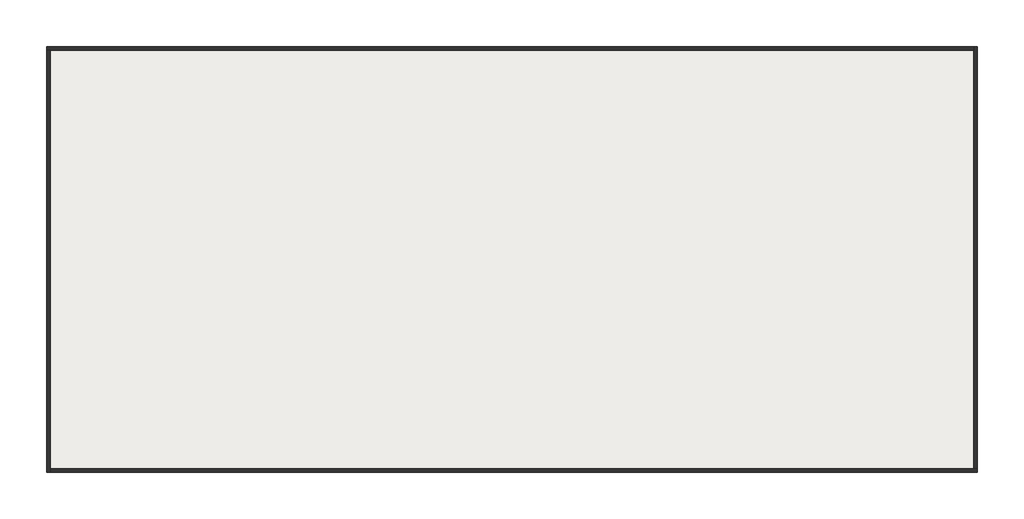
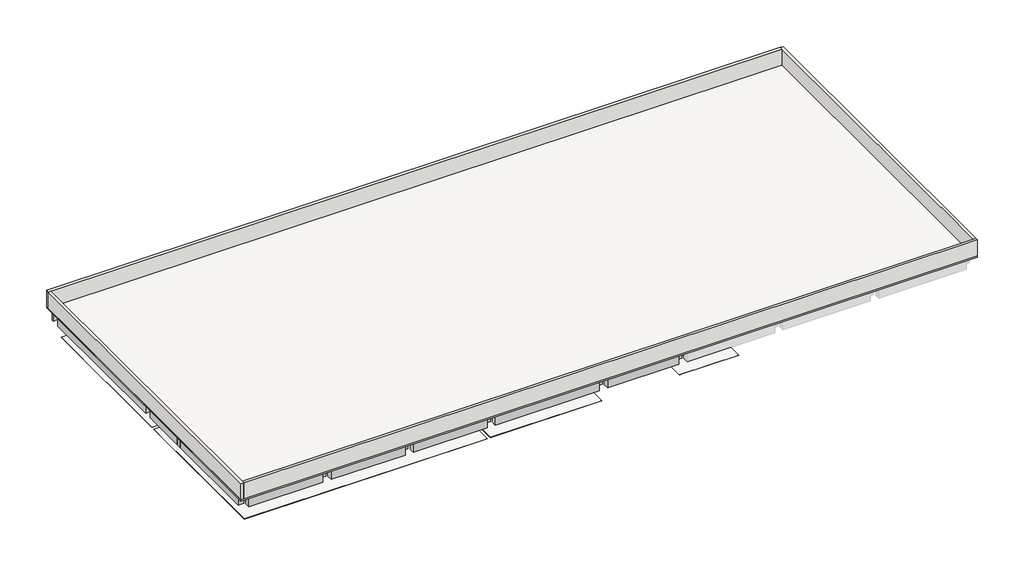
# One storey, part 1 of 2: 25 beams, 16 coverings, 4 walls, 1 roof.
"""IFC4 building model written with IfcOpenShell, lengths in millimetres."""

from ifc_helpers import new_model, si_unit, frame, origin, place, context, project, spatial, polyline, outline, extrude, faceted_brep, element, save

model = new_model("IFC4")

# Units and contexts
model_context = context("Model", 3, world=origin())
ifc_project = project(units=[si_unit("LENGTHUNIT", "METRE", prefix="MILLI")], contexts=[model_context])

# Site, building, storey
site = spatial("IfcSite", under=ifc_project)
building = spatial("IfcBuilding", under=site)
storey = spatial("IfcBuildingStorey", under=building, Name="TOC", Elevation=7650.0)

# Beams
placement = place(None, origin())
element("IfcBeam", 1, ObjectType="RC Beam_Rectangular : H_SB_ACB_B400xH900", at=placement, inside=storey, context=model_context, shape_type="Brep", body=[
    faceted_brep([(224.7, 12116.5208589, 7500.0), (224.7, 12116.5208589, 6750.0), (5624.7, 12116.5208589, 6750.0), (5624.7, 12116.5208589, 7500.0), (5724.7, 12116.5208589, 7500.0), (6124.7, 12116.5208589, 7500.0), (6124.7, 12116.5208589, 7549.0), (5724.7, 12116.5208589, 7549.0), (124.7, 12116.5208589, 7549.0), (-275.3, 12116.5208589, 7549.0), (-275.3, 12116.5208589, 7500.0), (124.7, 12116.5208589, 7500.0), (224.7, 12516.5208589, 6750.0), (5624.7, 12516.5208589, 6750.0), (224.7, 12516.5208589, 7500.0), (124.7, 12516.5208589, 7500.0), (-275.3, 12516.5208589, 7500.0), (-275.3, 12516.5208589, 7549.0), (124.7, 12516.5208589, 7549.0), (5724.7, 12516.5208589, 7549.0), (6124.7, 12516.5208589, 7549.0), (6124.7, 12516.5208589, 7500.0), (5724.7, 12516.5208589, 7500.0), (5624.7, 12516.5208589, 7500.0)], [[[0, 1, 2, 3, 4, 5, 6, 7, 8, 9, 10, 11]], [[1, 12, 13, 2]], [[12, 14, 15, 16, 17, 18, 19, 20, 21, 22, 23, 13]], [[1, 0, 14, 12]], [[0, 11, 10, 16, 15, 14]], [[23, 3, 2, 13]], [[3, 23, 22, 21, 5, 4]], [[9, 8, 7, 6, 20, 19, 18, 17]], [[9, 17, 16, 10]], [[20, 6, 5, 21]]]),
])
element("IfcBeam", 2, ObjectType="RC Beam_Rectangular : H_SB_ACB_B400xH900", at=placement, inside=storey, context=model_context, shape_type="Brep", body=[
    faceted_brep([(6224.7, 12116.5208589, 7500.0), (6224.7, 12116.5208589, 6750.0), (11624.7, 12116.5208589, 6750.0), (11624.7, 12116.5208589, 7500.0), (11724.7, 12116.5208589, 7500.0), (12124.7, 12116.5208589, 7500.0), (12124.7, 12116.5208589, 7549.0), (11724.7, 12116.5208589, 7549.0), (6124.7, 12116.5208589, 7549.0), (6124.7, 12116.5208589, 7500.0), (6224.7, 12516.5208589, 6750.0), (11624.7, 12516.5208589, 6750.0), (6224.7, 12516.5208589, 7500.0), (6124.7, 12516.5208589, 7500.0), (6124.7, 12516.5208589, 7549.0), (11724.7, 12516.5208589, 7549.0), (12124.7, 12516.5208589, 7549.0), (12124.7, 12516.5208589, 7500.0), (11724.7, 12516.5208589, 7500.0), (11624.7, 12516.5208589, 7500.0)], [[[0, 1, 2, 3, 4, 5, 6, 7, 8, 9]], [[1, 10, 11, 2]], [[10, 12, 13, 14, 15, 16, 17, 18, 19, 11]], [[1, 0, 12, 10]], [[0, 9, 13, 12]], [[19, 3, 2, 11]], [[3, 19, 18, 17, 5, 4]], [[8, 7, 6, 16, 15, 14]], [[16, 6, 5, 17]], [[8, 14, 13, 9]]]),
])
element("IfcBeam", 3, ObjectType="RC Beam_Rectangular : H_SB_ACB_B400xH900", at=placement, inside=storey, context=model_context, shape_type="Brep", body=[
    faceted_brep([(12224.7, 12116.5208589, 7500.0), (12224.7, 12116.5208589, 6750.0), (17624.7, 12116.5208589, 6750.0), (17624.7, 12116.5208589, 7500.0), (17724.7, 12116.5208589, 7500.0), (18124.7, 12116.5208589, 7500.0), (18124.7, 12116.5208589, 7549.0), (17724.7, 12116.5208589, 7549.0), (12124.7, 12116.5208589, 7549.0), (12124.7, 12116.5208589, 7500.0), (12224.7, 12516.5208589, 6750.0), (17624.7, 12516.5208589, 6750.0), (12224.7, 12516.5208589, 7500.0), (12124.7, 12516.5208589, 7500.0), (12124.7, 12516.5208589, 7549.0), (17724.7, 12516.5208589, 7549.0), (18124.7, 12516.5208589, 7549.0), (18124.7, 12516.5208589, 7500.0), (17724.7, 12516.5208589, 7500.0), (17624.7, 12516.5208589, 7500.0)], [[[0, 1, 2, 3, 4, 5, 6, 7, 8, 9]], [[1, 10, 11, 2]], [[10, 12, 13, 14, 15, 16, 17, 18, 19, 11]], [[1, 0, 12, 10]], [[0, 9, 13, 12]], [[19, 3, 2, 11]], [[3, 19, 18, 17, 5, 4]], [[8, 7, 6, 16, 15, 14]], [[16, 6, 5, 17]], [[8, 14, 13, 9]]]),
])
element("IfcBeam", 4, ObjectType="RC Beam_Rectangular : H_SB_ACB_B400xH900", at=placement, inside=storey, context=model_context, shape_type="Brep", body=[
    faceted_brep([(26324.7, 12116.5208589, 7549.0), (25924.7, 12116.5208589, 7549.0), (18124.7, 12116.5208589, 7549.0), (18124.7, 12116.5208589, 7500.0), (18224.7, 12116.5208589, 7500.0), (18224.7, 12116.5208589, 6750.0), (25924.7, 12116.5208589, 6750.0), (26324.7, 12116.5208589, 6750.0), (26324.7, 12516.5208589, 6750.0), (18224.7, 12516.5208589, 6750.0), (25924.7, 12516.5208589, 6750.0), (18124.7, 12516.5208589, 7549.0), (25924.7, 12516.5208589, 7549.0), (26324.7, 12516.5208589, 7549.0), (18224.7, 12516.5208589, 7500.0), (18124.7, 12516.5208589, 7500.0)], [[[0, 1, 2, 3, 4, 5, 6, 7]], [[8, 7, 6, 5, 9, 10]], [[11, 12, 13, 8, 10, 9, 14, 15]], [[4, 14, 9, 5]], [[14, 4, 3, 15]], [[2, 1, 0, 13, 12, 11]], [[7, 8, 13, 0]], [[2, 11, 15, 3]]]),
])
element("IfcBeam", 5, ObjectType="RC Beam_Rectangular : H_SB_ACB_B400xH900", at=placement, inside=storey, context=model_context, shape_type="Brep", body=[
    faceted_brep([(-275.3, 8216.5208589, 6750.0), (124.7, 8216.5208589, 6750.0), (5724.7, 8216.5208589, 6750.0), (6124.7, 8216.5208589, 6750.0), (6124.7, 8216.5208589, 7549.0), (5724.7, 8216.5208589, 7549.0), (124.7, 8216.5208589, 7549.0), (-275.3, 8216.5208589, 7549.0), (-275.3, 8616.5208589, 6750.0), (124.7, 8616.5208589, 6750.0), (5724.7, 8616.5208589, 6750.0), (6124.7, 8616.5208589, 6750.0), (-275.3, 8616.5208589, 7549.0), (124.7, 8616.5208589, 7549.0), (5724.7, 8616.5208589, 7549.0), (6124.7, 8616.5208589, 7549.0)], [[[0, 1, 2, 3, 4, 5, 6, 7]], [[0, 8, 9, 10, 11, 3, 2, 1]], [[11, 10, 9, 8, 12, 13, 14, 15]], [[7, 6, 5, 4, 15, 14, 13, 12]], [[8, 0, 7, 12]], [[3, 11, 15, 4]]]),
])
element("IfcBeam", 6, ObjectType="RC Beam_Rectangular : H_SB_ACB_B400xH900", at=placement, inside=storey, context=model_context, shape_type="Brep", body=[
    faceted_brep([(12124.7, 8216.5208589, 6750.0), (12124.7, 8216.5208589, 7549.0), (11724.7, 8216.5208589, 7549.0), (6124.7, 8216.5208589, 7549.0), (6124.7, 8216.5208589, 6750.0), (11724.7, 8216.5208589, 6750.0), (12124.7, 8616.5208589, 6750.0), (6124.7, 8616.5208589, 6750.0), (11724.7, 8616.5208589, 6750.0), (12124.7, 8616.5208589, 7549.0), (6124.7, 8616.5208589, 7549.0), (11724.7, 8616.5208589, 7549.0)], [[[0, 1, 2, 3, 4, 5]], [[6, 0, 5, 4, 7, 8]], [[9, 6, 8, 7, 10, 11]], [[1, 9, 11, 10, 3, 2]], [[0, 6, 9, 1]], [[4, 3, 10, 7]]]),
])
element("IfcBeam", 7, ObjectType="RC Beam_Rectangular : H_SB_ACB_B400xH900", at=placement, inside=storey, context=model_context, shape_type="Brep", body=[
    faceted_brep([(18124.7, 8216.5208589, 6750.0), (18124.7, 8216.5208589, 7549.0), (17724.7, 8216.5208589, 7549.0), (12124.7, 8216.5208589, 7549.0), (12124.7, 8216.5208589, 6750.0), (17724.7, 8216.5208589, 6750.0), (18124.7, 8616.5208589, 6750.0), (12124.7, 8616.5208589, 6750.0), (17724.7, 8616.5208589, 6750.0), (18124.7, 8616.5208589, 7549.0), (12124.7, 8616.5208589, 7549.0), (17724.7, 8616.5208589, 7549.0)], [[[0, 1, 2, 3, 4, 5]], [[6, 0, 5, 4, 7, 8]], [[9, 6, 8, 7, 10, 11]], [[1, 9, 11, 10, 3, 2]], [[0, 6, 9, 1]], [[4, 3, 10, 7]]]),
])
element("IfcBeam", 8, ObjectType="RC Beam_Rectangular : H_SB_ACB_B400xH900", at=placement, inside=storey, context=model_context, shape_type="Brep", body=[
    faceted_brep([(26324.7, 8216.5208589, 7549.0), (25924.7, 8216.5208589, 7549.0), (18124.7, 8216.5208589, 7549.0), (18124.7, 8216.5208589, 6750.0), (25824.7, 8216.5208589, 6750.0), (25824.7, 8216.5208589, 7500.0), (25924.7, 8216.5208589, 7500.0), (26324.7, 8216.5208589, 7500.0), (18124.7, 8616.5208589, 6750.0), (25824.7, 8616.5208589, 6750.0), (18124.7, 8616.5208589, 7549.0), (25924.7, 8616.5208589, 7549.0), (26324.7, 8616.5208589, 7549.0), (26324.7, 8616.5208589, 7500.0), (25924.7, 8616.5208589, 7500.0), (25824.7, 8616.5208589, 7500.0)], [[[0, 1, 2, 3, 4, 5, 6, 7]], [[3, 8, 9, 4]], [[10, 11, 12, 13, 14, 15, 9, 8]], [[15, 5, 4, 9]], [[5, 15, 14, 13, 7, 6]], [[2, 1, 0, 12, 11, 10]], [[12, 0, 7, 13]], [[3, 2, 10, 8]]]),
])
element("IfcBeam", 9, ObjectType="RC Beam_Rectangular : H_SB_ACB_B400xH900", at=placement, inside=storey, context=model_context, shape_type="Brep", body=[
    faceted_brep([(224.7, 416.5208589, 7500.0), (224.7, 416.5208589, 6750.0), (5624.7, 416.5208589, 6750.0), (5624.7, 416.5208589, 7500.0), (6124.7, 416.5208589, 7500.0), (6124.7, 416.5208589, 7549.0), (-275.3, 416.5208589, 7549.0), (-275.3, 416.5208589, 7500.0), (224.7, 816.5208589, 6750.0), (5624.7, 816.5208589, 6750.0), (224.7, 816.5208589, 7500.0), (124.7, 816.5208589, 7500.0), (-275.3, 816.5208589, 7500.0), (-275.3, 816.5208589, 7549.0), (124.7, 816.5208589, 7549.0), (5724.7, 816.5208589, 7549.0), (6124.7, 816.5208589, 7549.0), (6124.7, 816.5208589, 7500.0), (5724.7, 816.5208589, 7500.0), (5624.7, 816.5208589, 7500.0)], [[[0, 1, 2, 3, 4, 5, 6, 7]], [[1, 8, 9, 2]], [[8, 10, 11, 12, 13, 14, 15, 16, 17, 18, 19, 9]], [[8, 1, 0, 10]], [[12, 11, 10, 0, 7]], [[19, 3, 2, 9]], [[3, 19, 18, 17, 4]], [[6, 5, 16, 15, 14, 13]], [[6, 13, 12, 7]], [[16, 5, 4, 17]]]),
])
element("IfcBeam", 10, ObjectType="RC Beam_Rectangular : H_SB_ACB_B400xH900", at=placement, inside=storey, context=model_context, shape_type="Brep", body=[
    faceted_brep([(6224.7, 416.5208589, 7500.0), (6224.7, 416.5208589, 6750.0), (11624.7, 416.5208589, 6750.0), (11624.7, 416.5208589, 7500.0), (12124.7, 416.5208589, 7500.0), (12124.7, 416.5208589, 7549.0), (6124.7, 416.5208589, 7549.0), (6124.7, 416.5208589, 7500.0), (6224.7, 816.5208589, 6750.0), (11624.7, 816.5208589, 6750.0), (6224.7, 816.5208589, 7500.0), (6124.7, 816.5208589, 7500.0), (6124.7, 816.5208589, 7549.0), (11724.7, 816.5208589, 7549.0), (12124.7, 816.5208589, 7549.0), (12124.7, 816.5208589, 7500.0), (11724.7, 816.5208589, 7500.0), (11624.7, 816.5208589, 7500.0)], [[[0, 1, 2, 3, 4, 5, 6, 7]], [[1, 8, 9, 2]], [[8, 10, 11, 12, 13, 14, 15, 16, 17, 9]], [[8, 1, 0, 10]], [[11, 10, 0, 7]], [[17, 3, 2, 9]], [[3, 17, 16, 15, 4]], [[6, 5, 14, 13, 12]], [[14, 5, 4, 15]], [[6, 12, 11, 7]]]),
])
element("IfcBeam", 11, ObjectType="RC Beam_Rectangular : H_SB_ACB_B400xH900", at=placement, inside=storey, context=model_context, shape_type="Brep", body=[
    faceted_brep([(12224.7, 416.5208589, 7500.0), (12224.7, 416.5208589, 6750.0), (17624.7, 416.5208589, 6750.0), (17624.7, 416.5208589, 7500.0), (18124.7, 416.5208589, 7500.0), (18124.7, 416.5208589, 7549.0), (12124.7, 416.5208589, 7549.0), (12124.7, 416.5208589, 7500.0), (12224.7, 816.5208589, 6750.0), (17624.7, 816.5208589, 6750.0), (12224.7, 816.5208589, 7500.0), (12124.7, 816.5208589, 7500.0), (12124.7, 816.5208589, 7549.0), (17724.7, 816.5208589, 7549.0), (18124.7, 816.5208589, 7549.0), (18124.7, 816.5208589, 7500.0), (17724.7, 816.5208589, 7500.0), (17624.7, 816.5208589, 7500.0)], [[[0, 1, 2, 3, 4, 5, 6, 7]], [[1, 8, 9, 2]], [[8, 10, 11, 12, 13, 14, 15, 16, 17, 9]], [[8, 1, 0, 10]], [[11, 10, 0, 7]], [[17, 3, 2, 9]], [[3, 17, 16, 15, 4]], [[6, 5, 14, 13, 12]], [[14, 5, 4, 15]], [[6, 12, 11, 7]]]),
])
element("IfcBeam", 12, ObjectType="RC Beam_Rectangular : H_SB_ACB_B400xH900", at=placement, inside=storey, context=model_context, shape_type="Brep", body=[
    faceted_brep([(18224.7, 416.5208589, 7500.0), (18224.7, 416.5208589, 6750.0), (25824.7, 416.5208589, 6750.0), (25824.7, 416.5208589, 7500.0), (26324.7, 416.5208589, 7500.0), (26324.7, 416.5208589, 7549.0), (18124.7, 416.5208589, 7549.0), (18124.7, 416.5208589, 7500.0), (18224.7, 816.5208589, 6750.0), (25824.7, 816.5208589, 6750.0), (18224.7, 816.5208589, 7500.0), (18124.7, 816.5208589, 7500.0), (18124.7, 816.5208589, 7549.0), (25924.7, 816.5208589, 7549.0), (26324.7, 816.5208589, 7549.0), (26324.7, 816.5208589, 7500.0), (25924.7, 816.5208589, 7500.0), (25824.7, 816.5208589, 7500.0)], [[[0, 1, 2, 3, 4, 5, 6, 7]], [[1, 8, 9, 2]], [[8, 10, 11, 12, 13, 14, 15, 16, 17, 9]], [[8, 1, 0, 10]], [[11, 10, 0, 7]], [[17, 3, 2, 9]], [[3, 17, 16, 15, 4]], [[6, 5, 14, 13, 12]], [[14, 5, 4, 15]], [[6, 12, 11, 7]]]),
])
element("IfcBeam", 13, ObjectType="RC Beam_Rectangular : H_SB_ACB_B400xH900", at=placement, inside=storey, context=model_context, shape_type="Brep", body=[
    faceted_brep([(26424.7, 416.5208589, 7500.0), (26424.7, 416.5208589, 6750.0), (31624.7, 416.5208589, 6750.0), (31624.7, 416.5208589, 7500.0), (32124.7, 416.5208589, 7500.0), (32124.7, 416.5208589, 7549.0), (26324.7, 416.5208589, 7549.0), (26324.7, 416.5208589, 7500.0), (26424.7, 816.5208589, 6750.0), (31624.7, 816.5208589, 6750.0), (26424.7, 816.5208589, 7500.0), (26324.7, 816.5208589, 7500.0), (26324.7, 816.5208589, 7549.0), (31724.7, 816.5208589, 7549.0), (32124.7, 816.5208589, 7549.0), (32124.7, 816.5208589, 7500.0), (31724.7, 816.5208589, 7500.0), (31624.7, 816.5208589, 7500.0)], [[[0, 1, 2, 3, 4, 5, 6, 7]], [[1, 8, 9, 2]], [[8, 10, 11, 12, 13, 14, 15, 16, 17, 9]], [[8, 1, 0, 10]], [[11, 10, 0, 7]], [[17, 3, 2, 9]], [[3, 17, 16, 15, 4]], [[6, 5, 14, 13, 12]], [[14, 5, 4, 15]], [[6, 12, 11, 7]]]),
])
element("IfcBeam", 14, ObjectType="RC Beam_Rectangular : H_SB_ACB_B400xH900", at=placement, inside=storey, context=model_context, shape_type="SweptSolid", body=[
    extrude(outline(polyline([(8216.5208589, 7549.0), (8216.5208589, 6750.0), (916.5208589, 6750.0), (916.5208589, 7500.0), (816.5208589, 7500.0), (816.5208589, 7549.0), (8216.5208589, 7549.0)])), frame((-275.3, 0.0, 0.0), z_axis=(1.0, 0.0, 0.0), x_axis=(0.0, 1.0, 0.0)), (0.0, 0.0, 1.0), 400.0),
])
element("IfcBeam", 15, ObjectType="RC Beam_Rectangular : H_SB_ACB_B400xH900", at=placement, inside=storey, context=model_context, shape_type="SweptSolid", body=[
    extrude(outline(polyline([(8616.5208589, 7549.0), (12116.5208589, 7549.0), (12116.5208589, 7500.0), (12016.5208589, 7500.0), (12016.5208589, 6750.0), (8616.5208589, 6750.0), (8616.5208589, 7549.0)])), frame((-275.3, 0.0, 0.0), z_axis=(1.0, 0.0, 0.0), x_axis=(0.0, 1.0, 0.0)), (0.0, 0.0, 1.0), 400.0),
])
element("IfcBeam", 16, ObjectType="RC Beam_Rectangular : H_SB_ACB_B400xH900", at=placement, inside=storey, context=model_context, shape_type="Brep", body=[
    faceted_brep([(124.7, 24429.2208589, 6750.0), (-275.3, 24429.2208589, 6750.0), (-275.3, 24429.2208589, 7549.0), (124.7, 24429.2208589, 7549.0), (124.7, 12616.5208589, 7500.0), (124.7, 12616.5208589, 6750.0), (124.7, 23716.5208589, 6750.0), (124.7, 23716.5208589, 7500.0), (124.7, 23816.5208589, 7500.0), (124.7, 24216.5208589, 7500.0), (124.7, 24316.5208589, 7500.0), (124.7, 24316.5208589, 6750.0), (124.7, 24216.5208589, 7549.0), (124.7, 23816.5208589, 7549.0), (124.7, 12516.5208589, 7549.0), (124.7, 12516.5208589, 7500.0), (-275.3, 24316.5208589, 6750.0), (-275.3, 12616.5208589, 6750.0), (-275.3, 12616.5208589, 7500.0), (-275.3, 12516.5208589, 7500.0), (-275.3, 12516.5208589, 7549.0), (-275.3, 24316.5208589, 7500.0), (-275.3, 23716.5208589, 7500.0), (-275.3, 23716.5208589, 6750.0)], [[[0, 1, 2, 3]], [[4, 5, 6, 7, 8, 9, 10, 11, 0, 3, 12, 13, 14, 15]], [[1, 0, 11, 16]], [[17, 18, 19, 20, 2, 1, 16, 21, 22, 23]], [[19, 15, 14, 20]], [[5, 4, 18, 17]], [[4, 15, 19, 18]], [[22, 7, 6, 23]], [[7, 22, 21, 10, 9, 8]], [[3, 2, 20, 14, 13, 12]], [[10, 21, 16, 11]], [[5, 17, 23, 6]]]),
])
element("IfcBeam", 17, ObjectType="RC Beam_Rectangular : H_SB_ACB_B400xH900", at=placement, inside=storey, context=model_context, shape_type="SweptSolid", body=[
    extrude(outline(polyline([(8216.5208589, 7549.0), (8216.5208589, 6750.0), (916.5208589, 6750.0), (916.5208589, 7500.0), (816.5208589, 7500.0), (816.5208589, 7549.0), (8216.5208589, 7549.0)])), frame((5724.7, 0.0, 0.0), z_axis=(1.0, 0.0, 0.0), x_axis=(0.0, 1.0, 0.0)), (0.0, 0.0, 1.0), 400.0),
])
element("IfcBeam", 18, ObjectType="RC Beam_Rectangular : H_SB_ACB_B400xH900", at=placement, inside=storey, context=model_context, shape_type="SweptSolid", body=[
    extrude(outline(polyline([(8616.5208589, 6750.0), (8616.5208589, 7549.0), (12116.5208589, 7549.0), (12116.5208589, 7500.0), (12016.5208589, 7500.0), (12016.5208589, 6750.0), (8616.5208589, 6750.0)])), frame((5724.7, 0.0, 0.0), z_axis=(1.0, 0.0, 0.0), x_axis=(0.0, 1.0, 0.0)), (0.0, 0.0, 1.0), 400.0),
])
element("IfcBeam", 19, ObjectType="RC Beam_Rectangular : H_SB_ACB_B400xH900", at=placement, inside=storey, context=model_context, shape_type="SweptSolid", body=[
    extrude(outline(polyline([(8216.5208589, 7549.0), (8216.5208589, 6750.0), (916.5208589, 6750.0), (916.5208589, 7500.0), (816.5208589, 7500.0), (816.5208589, 7549.0), (8216.5208589, 7549.0)])), frame((11724.7, 0.0, 0.0), z_axis=(1.0, 0.0, 0.0), x_axis=(0.0, 1.0, 0.0)), (0.0, 0.0, 1.0), 400.0),
])
element("IfcBeam", 20, ObjectType="RC Beam_Rectangular : H_SB_ACB_B400xH900", at=placement, inside=storey, context=model_context, shape_type="SweptSolid", body=[
    extrude(outline(polyline([(8616.5208589, 6750.0), (8616.5208589, 7549.0), (12116.5208589, 7549.0), (12116.5208589, 7500.0), (12016.5208589, 7500.0), (12016.5208589, 6750.0), (8616.5208589, 6750.0)])), frame((11724.7, 0.0, 0.0), z_axis=(1.0, 0.0, 0.0), x_axis=(0.0, 1.0, 0.0)), (0.0, 0.0, 1.0), 400.0),
])
element("IfcBeam", 21, ObjectType="RC Beam_Rectangular : H_SB_ACB_B400xH900", at=placement, inside=storey, context=model_context, shape_type="SweptSolid", body=[
    extrude(outline(polyline([(8216.5208589, 7549.0), (8216.5208589, 6750.0), (916.5208589, 6750.0), (916.5208589, 7500.0), (816.5208589, 7500.0), (816.5208589, 7549.0), (8216.5208589, 7549.0)])), frame((17724.7, 0.0, 0.0), z_axis=(1.0, 0.0, 0.0), x_axis=(0.0, 1.0, 0.0)), (0.0, 0.0, 1.0), 400.0),
])
element("IfcBeam", 22, ObjectType="RC Beam_Rectangular : H_SB_ACB_B400xH900", at=placement, inside=storey, context=model_context, shape_type="SweptSolid", body=[
    extrude(outline(polyline([(8616.5208589, 6750.0), (8616.5208589, 7549.0), (12116.5208589, 7549.0), (12116.5208589, 7500.0), (12016.5208589, 7500.0), (12016.5208589, 6750.0), (8616.5208589, 6750.0)])), frame((17724.7, 0.0, 0.0), z_axis=(1.0, 0.0, 0.0), x_axis=(0.0, 1.0, 0.0)), (0.0, 0.0, 1.0), 400.0),
])
element("IfcBeam", 23, ObjectType="RC Beam_Rectangular : H_SB_ACB_B400xH900", at=placement, inside=storey, context=model_context, shape_type="SweptSolid", body=[
    extrude(outline(polyline([(8116.5208589, 7500.0), (8116.5208589, 6750.0), (916.5208589, 6750.0), (916.5208589, 7500.0), (816.5208589, 7500.0), (816.5208589, 7549.0), (8216.5208589, 7549.0), (8216.5208589, 7500.0), (8116.5208589, 7500.0)])), frame((25924.7, 0.0, 0.0), z_axis=(1.0, 0.0, 0.0), x_axis=(0.0, 1.0, 0.0)), (0.0, 0.0, 1.0), 400.0),
])
element("IfcBeam", 24, ObjectType="RC Beam_Rectangular : H_SB_ACB_B400xH900", at=placement, inside=storey, context=model_context, shape_type="SweptSolid", body=[
    extrude(outline(polyline([(12116.5208589, 7549.0), (12116.5208589, 6750.0), (8716.5208589, 6750.0), (8716.5208589, 7500.0), (8616.5208589, 7500.0), (8616.5208589, 7549.0), (12116.5208589, 7549.0)])), frame((25924.7, 0.0, 0.0), z_axis=(1.0, 0.0, 0.0), x_axis=(0.0, 1.0, 0.0)), (0.0, 0.0, 1.0), 400.0),
])
element("IfcBeam", 25, ObjectType="RC Beam_Rectangular : H_SB_ACB_B400xH900", at=placement, inside=storey, context=model_context, shape_type="SweptSolid", body=[
    extrude(outline(polyline([(8116.5208589, 7500.0), (8116.5208589, 6750.0), (916.5208589, 6750.0), (916.5208589, 7500.0), (816.5208589, 7500.0), (816.5208589, 7549.0), (8216.5208589, 7549.0), (8216.5208589, 7500.0), (8116.5208589, 7500.0)])), frame((31724.7, 0.0, 0.0), z_axis=(1.0, 0.0, 0.0), x_axis=(0.0, 1.0, 0.0)), (0.0, 0.0, 1.0), 400.0),
])

# Coverings
element("IfcCovering", 26, ObjectType="CE741_Acoustic Tiled Ceiling System_600x600x9t_T_bar", at=placement, inside=storey, context=model_context, shape_type="SweptSolid", body=[
    extrude(outline(polyline([(54.7, 23886.5208589), (17807.7, 23886.5208589), (17807.7, 12433.5208589), (54.7, 12433.5208589), (54.7, 23886.5208589)])), frame((0.0, 0.0, 5650.0), z_axis=(0.0, 0.0, 1.0), x_axis=(1.0, 0.0, 0.0)), (0.0, 0.0, 1.0), 9.0),
])
element("IfcCovering", 27, ObjectType="CE741_Acoustic Tiled Ceiling System_600x600x9t_T_bar", at=placement, inside=storey, context=model_context, shape_type="SweptSolid", body=[
    extrude(outline(polyline([(18041.7, 8533.5208589), (18041.7, 23886.5208589), (33157.7, 23886.5208589), (33157.7, 8533.5208589), (18041.7, 8533.5208589)])), frame((0.0, 0.0, 5650.0), z_axis=(0.0, 0.0, 1.0), x_axis=(1.0, 0.0, 0.0)), (0.0, 0.0, 1.0), 9.0),
])
element("IfcCovering", 28, ObjectType="CE741_Acoustic Tiled Ceiling System_600x600x9t_T_bar", at=placement, inside=storey, context=model_context, shape_type="SweptSolid", body=[
    extrude(outline(polyline([(54.7, 746.5208589), (54.7, 12199.5208589), (17807.7, 12199.5208589), (17807.7, 746.5208589), (54.7, 746.5208589)])), frame((0.0, 0.0, 5650.0), z_axis=(0.0, 0.0, 1.0), x_axis=(1.0, 0.0, 0.0)), (0.0, 0.0, 1.0), 9.0),
])
element("IfcCovering", 29, ObjectType="CE741_Acoustic Tiled Ceiling System_600x600x9t_T_bar", at=placement, inside=storey, context=model_context, shape_type="SweptSolid", body=[
    extrude(outline(polyline([(26190.7, 746.5208589), (18041.7, 746.5208589), (18041.7, 8299.5208589), (26190.7, 8299.5208589), (26190.7, 746.5208589)])), frame((0.0, 0.0, 5650.0), z_axis=(0.0, 0.0, 1.0), x_axis=(1.0, 0.0, 0.0)), (0.0, 0.0, 1.0), 9.0),
])
element("IfcCovering", 30, ObjectType="CE741_Acoustic Tiled Ceiling System_600x600x9t_T_bar", at=placement, inside=storey, context=model_context, shape_type="SweptSolid", body=[
    extrude(outline(polyline([(33391.7, 8533.5208589), (33391.7, 23886.5208589), (43607.7, 23886.5208589), (43607.7, 11083.5208589), (36207.7, 11083.5208589), (36207.7, 8533.5208589), (33391.7, 8533.5208589)])), frame((0.0, 0.0, 5650.0), z_axis=(0.0, 0.0, 1.0), x_axis=(1.0, 0.0, 0.0)), (0.0, 0.0, 1.0), 9.0),
])
element("IfcCovering", 31, ObjectType="CE741_Acoustic Tiled Ceiling System_600x600x9t_T_bar", at=placement, inside=storey, context=model_context, shape_type="SweptSolid", body=[
    extrude(outline(polyline([(54.7, 746.5208589), (54.7, 12199.5208589), (17807.7, 12199.5208589), (17807.7, 746.5208589), (54.7, 746.5208589)])), frame((0.0, 0.0, 5650.0), z_axis=(0.0, 0.0, 1.0), x_axis=(1.0, 0.0, 0.0)), (0.0, 0.0, 1.0), 9.0),
])
element("IfcCovering", 32, ObjectType="CE741_Acoustic Tiled Ceiling System_600x600x9t_T_bar", at=placement, inside=storey, context=model_context, shape_type="SweptSolid", body=[
    extrude(outline(polyline([(54.7, 23886.5208589), (17807.7, 23886.5208589), (17807.7, 12433.5208589), (54.7, 12433.5208589), (54.7, 23886.5208589)])), frame((0.0, 0.0, 5650.0), z_axis=(0.0, 0.0, 1.0), x_axis=(1.0, 0.0, 0.0)), (0.0, 0.0, 1.0), 9.0),
])
element("IfcCovering", 33, ObjectType="CE741_Acoustic Tiled Ceiling System_600x600x9t_T_bar", at=placement, inside=storey, context=model_context, shape_type="SweptSolid", body=[
    extrude(outline(polyline([(18041.7, 8533.5208589), (18041.7, 23886.5208589), (33157.7, 23886.5208589), (33157.7, 8533.5208589), (18041.7, 8533.5208589)])), frame((0.0, 0.0, 5650.0), z_axis=(0.0, 0.0, 1.0), x_axis=(1.0, 0.0, 0.0)), (0.0, 0.0, 1.0), 9.0),
])
element("IfcCovering", 34, ObjectType="CE741_Acoustic Tiled Ceiling System_600x600x9t_T_bar", at=placement, inside=storey, context=model_context, shape_type="SweptSolid", body=[
    extrude(outline(polyline([(26190.7, 746.5208589), (18041.7, 746.5208589), (18041.7, 8299.5208589), (26190.7, 8299.5208589), (26190.7, 746.5208589)])), frame((0.0, 0.0, 5650.0), z_axis=(0.0, 0.0, 1.0), x_axis=(1.0, 0.0, 0.0)), (0.0, 0.0, 1.0), 9.0),
])
element("IfcCovering", 35, ObjectType="CE741_Acoustic Tiled Ceiling System_600x600x9t_T_bar", at=placement, inside=storey, context=model_context, shape_type="SweptSolid", body=[
    extrude(outline(polyline([(26424.7, 2880.5208589), (26424.7, 8299.5208589), (28824.7, 8299.5208589), (28824.7, 2880.5208589), (26424.7, 2880.5208589)])), frame((0.0, 0.0, 5650.0), z_axis=(0.0, 0.0, 1.0), x_axis=(1.0, 0.0, 0.0)), (0.0, 0.0, 1.0), 9.0),
])
element("IfcCovering", 36, ObjectType="CE741_Acoustic Tiled Ceiling System_600x600x9t_T_bar", at=placement, inside=storey, context=model_context, shape_type="SweptSolid", body=[
    extrude(outline(polyline([(33391.7, 8533.5208589), (33391.7, 23886.5208589), (43607.7, 23886.5208589), (43607.7, 11083.5208589), (36207.7, 11083.5208589), (36207.7, 8533.5208589), (33391.7, 8533.5208589)])), frame((0.0, 0.0, 5650.0), z_axis=(0.0, 0.0, 1.0), x_axis=(1.0, 0.0, 0.0)), (0.0, 0.0, 1.0), 9.0),
])
element("IfcCovering", 37, ObjectType="CE741_Acoustic Tiled Ceiling System_600x600x9t_T_bar", at=placement, inside=storey, context=model_context, shape_type="SweptSolid", body=[
    extrude(outline(polyline([(38807.7, 3380.5208589), (36441.7, 3380.5208589), (36441.7, 10849.5208589), (45807.7, 10849.5208589), (45807.7, 9899.5208589), (49977.7, 9899.5208589), (49977.7, 10499.5208589), (50660.7, 10499.5208589), (50660.7, 8533.5208589), (45124.7, 8533.5208589), (45124.7, 8299.5208589), (45175.8778017, 8299.5208589), (45175.8778017, 6933.5208589), (43341.7, 6933.5208589), (43341.7, 8533.5208589), (38807.7, 8533.5208589), (38807.7, 3380.5208589)])), frame((0.0, 0.0, 5650.0), z_axis=(0.0, 0.0, 1.0), x_axis=(1.0, 0.0, 0.0)), (0.0, 0.0, 1.0), 9.0),
])
element("IfcCovering", 38, ObjectType="CE741_Acoustic Tiled Ceiling System_600x600x9t_T_bar", at=placement, inside=storey, context=model_context, shape_type="SweptSolid", body=[
    extrude(outline(polyline([(36207.7, 746.5208589), (31858.7, 746.5208589), (31858.7, 8299.5208589), (36207.7, 8299.5208589), (36207.7, 746.5208589)])), frame((0.0, 0.0, 5650.0), z_axis=(0.0, 0.0, 1.0), x_axis=(1.0, 0.0, 0.0)), (0.0, 0.0, 1.0), 9.0),
])
element("IfcCovering", 39, ObjectType="CE741_Acoustic Tiled Ceiling System_600x600x9t_T_bar", at=placement, inside=storey, context=model_context, shape_type="SweptSolid", body=[
    extrude(outline(polyline([(52794.7, 14049.5208589), (52794.7, 11967.5208589), (50660.7, 11967.5208589), (50660.7, 10733.5208589), (49743.7, 10733.5208589), (49743.7, 10133.5208589), (46041.7, 10133.5208589), (46041.7, 14049.5208589), (52794.7, 14049.5208589)])), frame((0.0, 0.0, 5650.0), z_axis=(0.0, 0.0, 1.0), x_axis=(1.0, 0.0, 0.0)), (0.0, 0.0, 1.0), 9.0),
])
element("IfcCovering", 40, ObjectType="CE741_Acoustic Tiled Ceiling System_600x600x9t_T_bar", at=placement, inside=storey, context=model_context, shape_type="SweptSolid", body=[
    extrude(outline(polyline([(52794.7, 18549.5208589), (52794.7, 14283.5208589), (48441.7, 14283.5208589), (48441.7, 17180.5208589), (46041.7, 17180.5208589), (46041.7, 18549.5208589), (52794.7, 18549.5208589)])), frame((0.0, 0.0, 5650.0), z_axis=(0.0, 0.0, 1.0), x_axis=(1.0, 0.0, 0.0)), (0.0, 0.0, 1.0), 9.0),
])
element("IfcCovering", 41, ObjectType="CE741_Acoustic Tiled Ceiling System_600x600x9t_T_bar", at=placement, inside=storey, context=model_context, shape_type="SweptSolid", body=[
    extrude(outline(polyline([(49041.7, 19949.5208589), (49041.7, 23886.5208589), (52794.7, 23886.5208589), (52794.7, 18783.5208589), (47658.7, 18783.5208589), (47658.7, 19949.5208589), (49041.7, 19949.5208589)])), frame((0.0, 0.0, 5650.0), z_axis=(0.0, 0.0, 1.0), x_axis=(1.0, 0.0, 0.0)), (0.0, 0.0, 1.0), 9.0),
])

# Roof
element("IfcRoof", 42, ObjectType="H_RF_AMF_RC Roof Finish_WP_Insulation_Protection", at=placement, inside=storey, context=model_context, shape_type="SweptSolid", body=[
    extrude(outline(polyline([(53324.7, 24816.5208589), (53324.7, 216.5208589), (-475.3, 216.5208589), (-475.3, 24816.5208589), (53324.7, 24816.5208589)])), frame((0.0, 0.0, 7549.0), z_axis=(0.0, 0.0, 1.0), x_axis=(1.0, 0.0, 0.0)), (0.0, 0.0, 1.0), 101.0),
])

# Walls
element("IfcWall", 43, ObjectType="H_WA_AMW_RC Wall_T200 (No Finish)", at=placement, inside=storey, context=model_context, shape_type="Brep", body=[
    faceted_brep([(-475.3, 24616.5208589, 7650.0), (-275.3, 24616.5208589, 7650.0), (53124.7, 24616.5208589, 7650.0), (53124.7, 24616.5208589, 8900.0), (-275.3, 24616.5208589, 8900.0), (-475.3, 24616.5208589, 8900.0), (-475.3, 24816.5208589, 7650.0), (-475.3, 24816.5208589, 8900.0), (53124.7, 24816.5208589, 8900.0), (53124.7, 24816.5208589, 7650.0)], [[[0, 1, 2, 3, 4, 5]], [[6, 7, 8, 9]], [[2, 1, 0, 6, 9]], [[5, 4, 3, 8, 7]], [[0, 5, 7, 6]], [[3, 2, 9, 8]]]),
])
element("IfcWall", 44, ObjectType="H_WA_AMW_RC Wall_T200 (No Finish)", at=placement, inside=storey, context=model_context, shape_type="Brep", body=[
    faceted_brep([(-275.3, 216.5208589, 7650.0), (-275.3, 416.5208589, 7650.0), (-275.3, 24616.5208589, 7650.0), (-275.3, 24616.5208589, 8900.0), (-275.3, 416.5208589, 8900.0), (-275.3, 216.5208589, 8900.0), (-475.3, 216.5208589, 7650.0), (-475.3, 216.5208589, 8900.0), (-475.3, 24616.5208589, 8900.0), (-475.3, 24616.5208589, 7650.0)], [[[0, 1, 2, 3, 4, 5]], [[6, 7, 8, 9]], [[2, 1, 0, 6, 9]], [[5, 4, 3, 8, 7]], [[0, 5, 7, 6]], [[3, 2, 9, 8]]]),
])
element("IfcWall", 45, ObjectType="H_WA_AMW_RC Wall_T200 (No Finish)", at=placement, inside=storey, context=model_context, shape_type="Brep", body=[
    faceted_brep([(53324.7, 416.5208589, 7650.0), (53124.7, 416.5208589, 7650.0), (-275.3, 416.5208589, 7650.0), (-275.3, 416.5208589, 8900.0), (53124.7, 416.5208589, 8900.0), (53324.7, 416.5208589, 8900.0), (53324.7, 216.5208589, 7650.0), (53324.7, 216.5208589, 8900.0), (-275.3, 216.5208589, 8900.0), (-275.3, 216.5208589, 7650.0)], [[[0, 1, 2, 3, 4, 5]], [[6, 7, 8, 9]], [[2, 1, 0, 6, 9]], [[5, 4, 3, 8, 7]], [[0, 5, 7, 6]], [[3, 2, 9, 8]]]),
])
element("IfcWall", 46, ObjectType="H_WA_AMW_RC Wall_T200 (No Finish)", at=placement, inside=storey, context=model_context, shape_type="Brep", body=[
    faceted_brep([(53124.7, 24816.5208589, 7650.0), (53124.7, 24616.5208589, 7650.0), (53124.7, 416.5208589, 7650.0), (53124.7, 416.5208589, 8900.0), (53124.7, 24616.5208589, 8900.0), (53124.7, 24816.5208589, 8900.0), (53324.7, 24816.5208589, 7650.0), (53324.7, 24816.5208589, 8900.0), (53324.7, 416.5208589, 8900.0), (53324.7, 416.5208589, 7650.0)], [[[0, 1, 2, 3, 4, 5]], [[6, 7, 8, 9]], [[2, 1, 0, 6, 9]], [[5, 4, 3, 8, 7]], [[0, 5, 7, 6]], [[3, 2, 9, 8]]]),
])

save(model, "model.ifc")

# Revit data of these elements
# Project information
#   Building Name = "SULFUR LOADING CONTROL BD"
#   Project Status = "Project Status"
#   Client Name = "현대엔지니어링"
#   Project Address = "서울시 종로구 율곡로 75(계동)"
#   Project Number = "-"
# Grids (mm)
#   "Y1": line (-3935.398, 24016.521) -> (58968.688, 24016.521)
#   "X1": line (-75.3, 29394.337) -> (-75.3, -4379.638)
#   "X2": line (5924.7, 29394.337) -> (5924.7, -4379.638)
#   "Y3": line (-3935.398, 8416.521) -> (58968.688, 8416.521)
#   "Y4": line (-3935.398, 616.521) -> (58968.688, 616.521)
#   "X3": line (11924.7, 29394.337) -> (11924.7, -4379.638)
#   "X4": line (17924.7, 29394.337) -> (17924.7, -4379.638)
#   "X5": line (26124.7, 29394.337) -> (26124.7, -4379.638)
#   "X6": line (31924.7, 29394.337) -> (31924.7, -4379.638)
#   "X7": line (38924.7, 29394.337) -> (38924.7, -4379.638)
#   "X8": line (45924.7, 29394.337) -> (45924.7, -4379.638)
#   "X9": line (52924.7, 29394.337) -> (52924.7, -4379.638)
#   "X15": line (43724.7, 27041.858) -> (43724.7, 9156.488)
#   "X16": line (36324.7, 27041.858) -> (36324.7, 9156.488)
#   "X17": line (34685.051, 10966.521) -> (55094.626, 10966.521)
#   "X18": line (34685.051, 18666.521) -> (55094.626, 18666.521)
#   "Y2": line (-3935.398, 12316.521) -> (58968.688, 12316.521)
# Type "RC Beam_Rectangular : H_SB_ACB_B400xH900"
#   중앙부 하부근 = ""
#   중앙부 상부근 = ""
#   중앙부 보조근 = ""
#   중앙부 늑근 = ""
#   외단부 하부근 = ""
#   외단부 상부근 = ""
#   외단부 보조근 = ""
#   외단부 늑근 = ""
#   부호 = "TG3"
#   내단부 하부근 = ""
#   내단부 상부근 = ""
#   내단부 보조근 = ""
#   내단부 늑근 = ""
#   ALL 하부근 = "3-D20"
#   ALL 상부근 = "3-D20"
#   ALL 보조근 = ""
#   ALL 늑근 = "2-D10 @120"
#   Width = 400.000 mm
#   Height = 900.000 mm
#   Length [instance default] = 1524.000 mm
#   b = 400.000 mm
#   h = 900.000 mm
#   hec_material3 [instance default] = none
#   hec_material2 [instance default] = none
#   hec_material1 [instance default] = none
#   Structural Material [instance default] = none
#   Assembly Code = ""
# Type "CE741_Acoustic Tiled Ceiling System_600x600x9t_T_bar"
#   built-in parameter 1002203 = 1 (stored number, unit not read)
#   built-in parameter 1002202 = 1 (stored number, unit not read)
#   Layers, outside or top first: 9.000 mm no material (function 4)
# Type "H_RF_AMF_RC Roof Finish_WP_Insulation_Protection"
#   Layers, outside or top first: 50.000 mm no material (function 4); 0.000 mm no material (function 100); 50.000 mm no material (function 3); 1.000 mm no material (function 2)
# Type "H_WA_AMW_RC Wall_T200 (No Finish)"
#   Type Comments = ""
#   Layers, outside or top first: 0.000 mm no material (function 100); 0.000 mm no material (function 100); 200.000 mm no material (function 1); 0.000 mm no material (function 100); 0.000 mm no material (function 100); 0.000 mm no material (function 100)
# Elements 1, 2, 3, 4, 5, 6, 7, 8, 9, 10, 11, 12, 13, 14, 15, 16, 17, 18, 19, 20, 21, 22, 23, 24, 25 (IfcBeam, "RC Beam_Rectangular : H_SB_ACB_B400xH900")
#   hec_material3 = none
#   hec_material2 = none
#   hec_material1 = none
#   Structural Material = none
#   Phase Created = New Construction
# Elements 26, 27, 28, 29, 30, 31, 32, 33, 34, 35, 36, 37, 38, 39, 40, 41 (IfcCovering, "CE741_Acoustic Tiled Ceiling System_600x600x9t_T_bar")
#   Height Offset From Level = -2000.000 mm
#   Phase Created = New Construction
# Element 42 (IfcRoof, "H_RF_AMF_RC Roof Finish_WP_Insulation_Protection")
#   Mark = "RF1"
#   Roof Style Name = "Lightweight Concrete(Slope)+Insulation+Waterproofing+Gravel"
#   Roof Ref. = ""
#   Roof Base Material = "Concrete Slab"
#   Roof Finish_1 = "Light-Weight Concrete Screed (Slope 1%)"
#   Roof Finish_2 = ""
#   Roof Finish_3 = "Rigid Extruded Polystyrene Foam Insulation(XPS)"
#   Roof Finish_4 = "Waterproofing Membrane-EPDM(or Equivalent)"
#   Roof Finish_5 = "Gravel for Roof"
#   built-in parameter 1001705 = 25.0984 (stored number, unit not read)
#   built-in parameter 1001701 = -0.331365 (stored number, unit not read)
#   built-in parameter 1001710 = 33615
#   Roof Style = RF13
#   Phase Created = New Construction
#   Materials on its faces: "Default Roof"
# Element 43 (IfcWall, "H_WA_AMW_RC Wall_T200 (No Finish)")
#   Mark = "PW1"
#   Wall Loca = "ROOF"
#   Wall Style Name = "Concrete Wall+Acrylic Emulsion Paint on Cement Plaster"
#   Wall Ref. = ""
#   Wall Base Material-1 = ""
#   Wall Base Material-2 = ""
#   Wall Base Material-3 = "Concrete Wall"
#   Wall Finish-Ex = "Acrylic Emulsion Paint on Fair Faced Concrete"
#   Top Offset = 0.000 mm
#   Base Offset = 0.000 mm
#   wall height = 1250.000 mm
#   Wall Style No = EW51
#   Phase Created = New Construction
#   Base Constraint = TOC
#   Top Constraint = TOP
#   Materials on its faces: "Default Wall"
# Element 44 (IfcWall, "H_WA_AMW_RC Wall_T200 (No Finish)")
#   Mark = "PW2"
#   Wall Loca = "ROOF"
#   Wall Style Name = "Concrete Wall+Acrylic Emulsion Paint on Cement Plaster"
#   Wall Ref. = ""
#   Wall Base Material-1 = ""
#   Wall Base Material-2 = ""
#   Wall Base Material-3 = "Concrete Wall"
#   Wall Finish-Ex = "Acrylic Emulsion Paint on Fair Faced Concrete"
#   Top Offset = 0.000 mm
#   Base Offset = 0.000 mm
#   wall height = 1250.000 mm
#   Wall Style No = EW51
#   Phase Created = New Construction
#   Base Constraint = TOC
#   Top Constraint = TOP
#   Materials on its faces: "Default Wall"
# Element 45 (IfcWall, "H_WA_AMW_RC Wall_T200 (No Finish)")
#   Mark = "PW3"
#   Wall Loca = "ROOF"
#   Wall Style Name = "Concrete Wall+Acrylic Emulsion Paint on Cement Plaster"
#   Wall Ref. = ""
#   Wall Base Material-1 = ""
#   Wall Base Material-2 = ""
#   Wall Base Material-3 = "Concrete Wall"
#   Wall Finish-Ex = "Acrylic Emulsion Paint on Fair Faced Concrete"
#   Top Offset = 0.000 mm
#   Base Offset = 0.000 mm
#   wall height = 1250.000 mm
#   Wall Style No = EW51
#   Phase Created = New Construction
#   Base Constraint = TOC
#   Top Constraint = TOP
#   Materials on its faces: "Default Wall"
# Element 46 (IfcWall, "H_WA_AMW_RC Wall_T200 (No Finish)")
#   Mark = "PW4"
#   Wall Loca = "ROOF"
#   Wall Style Name = "Concrete Wall+Acrylic Emulsion Paint on Cement Plaster"
#   Wall Ref. = ""
#   Wall Base Material-1 = ""
#   Wall Base Material-2 = ""
#   Wall Base Material-3 = "Concrete Wall"
#   Wall Finish-Ex = "Acrylic Emulsion Paint on Fair Faced Concrete"
#   Top Offset = 0.000 mm
#   Base Offset = 0.000 mm
#   wall height = 1250.000 mm
#   Wall Style No = EW51
#   Phase Created = New Construction
#   Base Constraint = TOC
#   Top Constraint = TOP
#   Materials on its faces: "Default Wall"
# Materials
#   "Default Roof": class "Miscellaneous", colour RGB 80 80 80, transparency 0
#   "Default Wall": class "Miscellaneous", colour RGB 80 80 80, transparency 0
